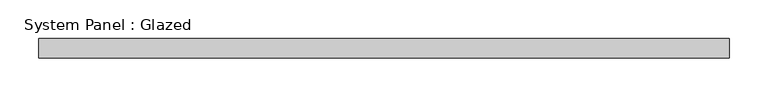
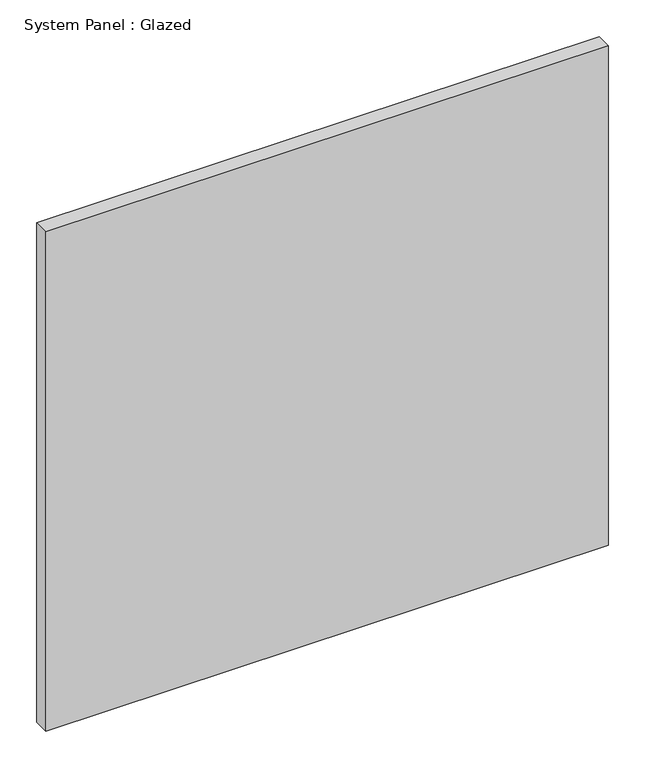
"""IFC4 building model written with IfcOpenShell, lengths in millimetres: plate geometry, System Panel : Glazed."""

from ifc_helpers import new_model, si_unit, origin, origin_with_axes, place, context, project, spatial, polyline, outline, extrude, source, transform, mapped, element, save


def system_panel_glazed_e5ed80d7(model_context):
    return source(origin(), model_context, "Body", "SweptSolid", [
        extrude(outline(polyline([(443.9393939, 24.5), (-443.9393939, 24.5), (-443.9393939, 49.5), (443.9393939, 49.5), (443.9393939, 24.5)])), origin_with_axes(), (0.0, 0.0, 1.0), 833.3333333),
    ])


if __name__ == "__main__":
    model = new_model("IFC4")
    model_context = context("Model", 3, world=origin())
    ifc_project = project(units=[si_unit("LENGTHUNIT", "METRE", prefix="MILLI")], contexts=[model_context])
    site = spatial("IfcSite", under=ifc_project)
    building = spatial("IfcBuilding", under=site)
    placement = place(None, origin())
    system_panel_glazed_shape = system_panel_glazed_e5ed80d7(model_context)
    element("IfcPlate", 1, ObjectType="System Panel : Glazed", at=placement, inside=building, context=model_context, shape_type="MappedRepresentation", body=[
        mapped(system_panel_glazed_shape, transform((0.0, 0.0, 0.0), x_axis=(1.0, 0.0, 0.0), y_axis=(0.0, 1.0, 0.0), z_axis=(0.0, 0.0, 1.0))),
    ])
    save(model, "model.ifc")

# Revit data of these elements
# Element 1 (IfcPlate, "System Panel : Glazed")
#   Materials on its faces: "Glass"
# Materials
#   "Glass": class "Glass", colour RGB 218 227 224, transparency 0.85, Description = "Soda Lime Glass", Cost = 0
